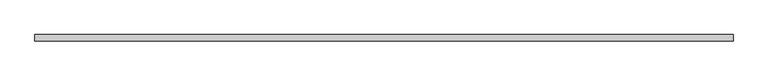
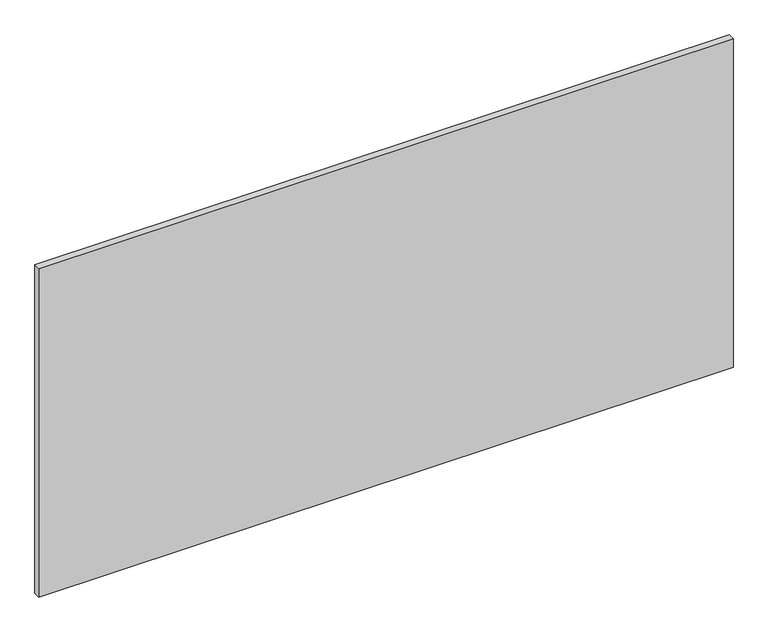
"""IFC4 building model written with IfcOpenShell, lengths in millimetres: proxy geometry, Inner panel:Inner panel:1:Inner panel:1 : Inner panel:Inner panel:300324:300043:Inner panel:1:Inner panel:1 : Inner panel:Inner panel:300324:300043 : Inner panel:Inner panel:1:Inner panel:1 : Inner panel:Inner panel:300324:300043:6 : Inner panel:Inner panel:1:Inner panel:1 : Inner panel:Inner panel:300324:300043:Inner panel:1:Inner panel:1 : Inner panel:Inner panel:300324:300043 : Inner panel:Inner panel:1:Inner panel:1 : Inner panel:Inner panel:300324:300043:300031."""

from ifc_helpers import new_model, si_unit, frame, origin, place, context, project, spatial, polyline, outline, extrude, source, transform, mapped, element, save


def generic_models_d6d41839(model_context):
    return source(origin(), model_context, "Body", "SweptSolid", [
        extrude(outline(polyline([(570452.6367239, -579000.6913841), (572891.0367239, -579000.6913841), (572891.0367239, -579022.9163841), (570452.6367239, -579022.9163841), (570452.6367239, -579000.6913841)])), frame((0.0, 0.0, 44.45), z_axis=(0.0, 0.0, 1.0), x_axis=(1.0, 0.0, 0.0)), (0.0, 0.0, 1.0), 1219.2),
    ])


if __name__ == "__main__":
    model = new_model("IFC4")
    model_context = context("Model", 3, world=origin())
    ifc_project = project(units=[si_unit("LENGTHUNIT", "METRE", prefix="MILLI")], contexts=[model_context])
    site = spatial("IfcSite", under=ifc_project)
    building = spatial("IfcBuilding", under=site)
    placement = place(None, origin())
    generic_models_shape = generic_models_d6d41839(model_context)
    element("IfcBuildingElementProxy", 1, Name="Inner panel:Inner panel:1:Inner panel:1 : Inner panel:Inner panel:300324:300043:Inner panel:1:Inner panel:1 : Inner panel:Inner panel:300324:300043 : Inner panel:Inner panel:1:Inner panel:1 : Inner panel:Inner panel:300324:300043:6 : Inner panel:Inner panel:1:Inner panel:1 : Inner panel:Inner panel:300324:300043:Inner panel:1:Inner panel:1 : Inner panel:Inner panel:300324:300043 : Inner panel:Inner panel:1:Inner panel:1 : Inner panel:Inner panel:300324:300043:300031", ObjectType="Inner panel:Inner panel:1:Inner panel:1 : Inner panel:Inner panel:300324:300043:Inner panel:1:Inner panel:1 : Inner panel:Inner panel:300324:300043 : Inner panel:Inner panel:1:Inner panel:1 : Inner panel:Inner panel:300324:300043:6 : Inner panel:Inner panel:1:Inner panel:1 : Inner panel:Inner panel:300324:300043:Inner panel:1:Inner panel:1 : Inner panel:Inner panel:300324:300043 : Inner panel:Inner panel:1:Inner panel:1 : Inner panel:Inner panel:300324:300043:300031", at=placement, inside=building, context=model_context, shape_type="MappedRepresentation", body=[
        mapped(generic_models_shape, transform((0.0, 0.0, 0.0), x_axis=(1.0, 0.0, 0.0), y_axis=(0.0, 1.0, 0.0), z_axis=(0.0, 0.0, 1.0))),
    ])
    save(model, "model.ifc")

# Revit data of these elements
# Type "Inner panel:Inner panel:1:Inner panel:1 : Inner panel:Inner panel:300324:300043:Inner panel:1:Inner panel:1 : Inner panel:Inner panel:300324:300043 : Inner panel:Inner panel:1:Inner panel:1 : Inner panel:Inner panel:300324:300043:6 : Inner panel:Inner panel:1:Inner panel:1 : Inner panel:Inner panel:300324:300043:Inner panel:1:Inner panel:1 : Inner panel:Inner panel:300324:300043 : Inner panel:Inner panel:1:Inner panel:1 : Inner panel:Inner panel:300324:300043:300031"
#   NameOverride = "Inner panel:Inner panel:1:Inner panel:1 : Inner panel:Inner panel:300324:300043:Inner panel:1:Inner panel:1 : Inner panel:Inner panel:300324:300043 : Inner panel:Inner panel:1:Inner panel:1 : Inner panel:Inner panel:300324:300043:300031"
#   ObjectTypeOverride = "Inner panel:1:Inner panel:1 : Inner panel:Inner panel:300324:300043 : Inner panel:Inner panel:1:Inner panel:1 : Inner panel:Inner panel:300324:300043"
#   Reference = "Inner panel"
#   Tag = "300031"
# Element 1 (IfcBuildingElementProxy, "Inner panel:Inner panel:1:Inner panel:1 : Inner panel:Inner panel:300324:300043:Inner panel:1:Inner panel:1 : Inner panel:Inner panel:300324:300043 : Inner panel:Inner panel:1:Inner panel:1 : Inner panel:Inner panel:300324:300043:6 : Inner panel:Inner panel:1:Inner panel:1 : Inner panel:Inner panel:300324:300043:Inner panel:1:Inner panel:1 : Inner panel:Inner panel:300324:300043 : Inner panel:Inner panel:1:Inner panel:1 : Inner panel:Inner panel:300324:300043:300031")
#   Materials on its faces: "1/2\" EXTERIOR GRADE FIRE RETARDANT CDX PLYWOOD"
# Materials
#   "1/2\" EXTERIOR GRADE FIRE RETARDANT CDX PLYWOOD": class "Unassigned", colour RGB 196 177 123, transparency 0, Cost = 0
